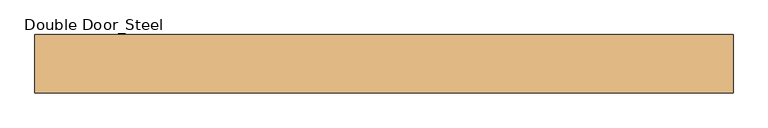
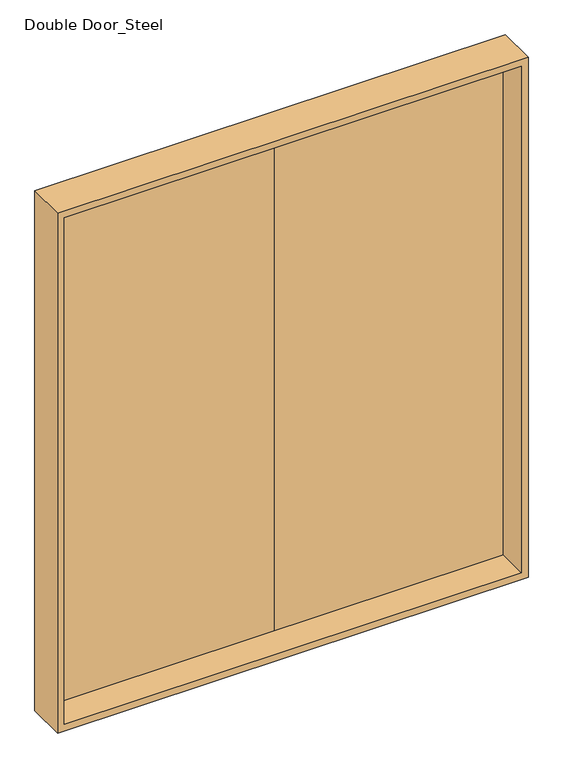
"""IFC4 building model written with IfcOpenShell, lengths in millimetres: door geometry, Double Door_Steel : H_DR_AR_B12_Double Door_Steel_W2400xH2800."""

from ifc_helpers import new_model, si_unit, frame, origin, place, context, project, spatial, polyline, outline, extrude, faceted_brep, source, transform, mapped, element, save


def double_door_steel_3c26782d(model_context):
    return source(origin(), model_context, "Body", "SolidModel", [
        extrude(outline(polyline([(1180.0, 60.0), (0.0, 60.0), (0.0, 100.0), (1180.0, 100.0), (1180.0, 60.0)])), frame((0.0, 0.0, 20.0), z_axis=(0.0, 0.0, 1.0), x_axis=(1.0, 0.0, 0.0)), (0.0, 0.0, 1.0), 2760.0),
        extrude(outline(polyline([(0.0, 60.0), (-1180.0, 60.0), (-1180.0, 100.0), (0.0, 100.0), (0.0, 60.0)])), frame((0.0, 0.0, 20.0), z_axis=(0.0, 0.0, 1.0), x_axis=(1.0, 0.0, 0.0)), (0.0, 0.0, 1.0), 2760.0),
        faceted_brep([(1200.0, -100.0, 2800.0), (1200.0, 100.0, 2800.0), (-1200.0, 100.0, 2800.0), (-1200.0, -100.0, 2800.0), (1165.0, 60.0, 2765.0), (1165.0, -100.0, 2765.0), (-1165.0, -100.0, 2765.0), (-1165.0, 60.0, 2765.0), (1180.0, 100.0, 2780.0), (1180.0, 60.0, 2780.0), (-1180.0, 60.0, 2780.0), (-1180.0, 100.0, 2780.0), (-1200.0, 100.0, 0.0), (-1200.0, -100.0, 0.0), (-1165.0, -100.0, 35.0), (-1165.0, 60.0, 35.0), (-1180.0, 60.0, 20.0), (-1180.0, 100.0, 20.0), (1200.0, 100.0, 0.0), (1180.0, 100.0, 20.0), (1200.0, -100.0, 0.0), (1165.0, -100.0, 35.0), (1165.0, 60.0, 35.0), (1180.0, 60.0, 20.0)], [[[0, 1, 2, 3]], [[4, 5, 6, 7]], [[8, 9, 10, 11]], [[3, 2, 12, 13]], [[7, 6, 14, 15]], [[11, 10, 16, 17]], [[18, 12, 2, 1], [8, 11, 17, 19]], [[13, 12, 18, 20]], [[0, 3, 13, 20], [21, 14, 6, 5]], [[15, 14, 21, 22]], [[23, 16, 10, 9], [4, 7, 15, 22]], [[17, 16, 23, 19]], [[20, 18, 1, 0]], [[22, 21, 5, 4]], [[19, 23, 9, 8]]]),
    ])


if __name__ == "__main__":
    model = new_model("IFC4")
    model_context = context("Model", 3, world=origin())
    ifc_project = project(units=[si_unit("LENGTHUNIT", "METRE", prefix="MILLI")], contexts=[model_context])
    site = spatial("IfcSite", under=ifc_project)
    building = spatial("IfcBuilding", under=site)
    placement = place(None, origin())
    double_door_steel_shape = double_door_steel_3c26782d(model_context)
    element("IfcDoor", 1, ObjectType="Double Door_Steel : H_DR_AR_B12_Double Door_Steel_W2400xH2800", at=placement, inside=building, context=model_context, shape_type="MappedRepresentation", body=[
        mapped(double_door_steel_shape, transform((0.0, 0.0, 0.0), x_axis=(1.0, 0.0, 0.0), y_axis=(0.0, 1.0, 0.0), z_axis=(0.0, 0.0, 1.0))),
    ])
    save(model, "model.ifc")

# Revit data of these elements
# Type "Double Door_Steel : H_DR_AR_B12_Double Door_Steel_W2400xH2800"
#   Type Mark = "429"
#   프레임 = ""
#   철물 = ""
#   유리/마감 = ""
#   위치/개소 = ""
#   부호 = "1/SD"
#   문번호 = ""
#   문기호 = "SD"
#   Analytic Construction = "<None>"
#   Height = 2800 mm
#   Width = 2400 mm
#   Define Thermal Properties by = 1
#   문 틀 = none
#   문 = none
#   Function = (empty or 0)
#   Assembly Code = ""
#   Wall Closure = (empty or 0)
